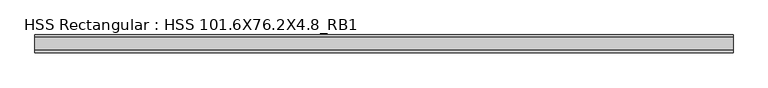
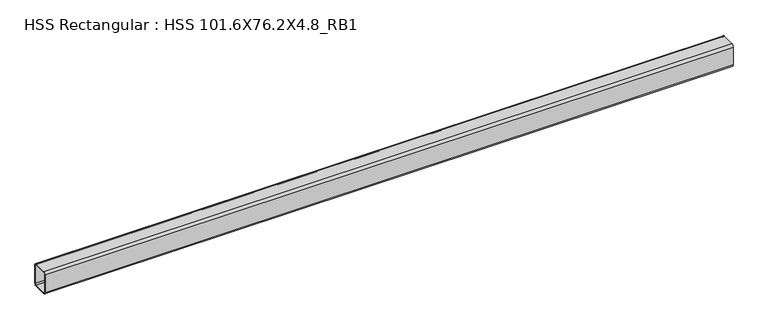
"""IFC4 building model written with IfcOpenShell, lengths in millimetres: beam geometry, HSS Rectangular : HSS 101.6X76.2X4.8_RB1."""

from ifc_helpers import new_model, si_unit, point, frame, frame_2d, origin, place, context, project, spatial, polyline, circle_curve, trimmed, segment, composite_curve, outline, extrude, source, transform, mapped, element, save


def hss_rectangular_hss_101_6x76_2x4_8_rb1_0456b7c3(model_context):
    return source(origin(), model_context, "Body", "SweptSolid", [
        extrude(outline(composite_curve([segment(trimmed(circle_curve(frame_2d((-28.575, 41.275)), 9.525), [point((-38.1, 41.275))], [point((-28.575, 50.8))], False, "CARTESIAN"), True, "CONTINUOUS"), segment(polyline([(-28.575, 50.8), (28.575, 50.8)]), True, "CONTINUOUS"), segment(trimmed(circle_curve(frame_2d((28.575, 41.275)), 9.525), [point((28.575, 50.8))], [point((38.1, 41.275))], False, "CARTESIAN"), True, "CONTINUOUS"), segment(polyline([(38.1, 41.275), (38.1, -41.275)]), True, "CONTINUOUS"), segment(trimmed(circle_curve(frame_2d((28.575, -41.275)), 9.525), [point((38.1, -41.275))], [point((28.575, -50.8))], False, "CARTESIAN"), True, "CONTINUOUS"), segment(polyline([(28.575, -50.8), (-28.575, -50.8)]), True, "CONTINUOUS"), segment(trimmed(circle_curve(frame_2d((-28.575, -41.275)), 9.525), [point((-28.575, -50.8))], [point((-38.1, -41.275))], False, "CARTESIAN"), True, "CONTINUOUS"), segment(polyline([(-38.1, -41.275), (-38.1, 41.275)]), True, "CONTINUOUS")], self_intersect=False), holes=[composite_curve([segment(polyline([(28.575, 46.0375), (-28.575, 46.0375)]), True, "CONTINUOUS"), segment(trimmed(circle_curve(frame_2d((-28.575, 41.275)), 4.7625), [point((-28.575, 46.0375))], [point((-33.3375, 41.275))], True, "CARTESIAN"), True, "CONTINUOUS"), segment(polyline([(-33.3375, 41.275), (-33.3375, -41.275)]), True, "CONTINUOUS"), segment(trimmed(circle_curve(frame_2d((-28.575, -41.275)), 4.7625), [point((-33.3375, -41.275))], [point((-28.575, -46.0375))], True, "CARTESIAN"), True, "CONTINUOUS"), segment(polyline([(-28.575, -46.0375), (28.575, -46.0375)]), True, "CONTINUOUS"), segment(trimmed(circle_curve(frame_2d((28.575, -41.275)), 4.7625), [point((28.575, -46.0375))], [point((33.3375, -41.275))], True, "CARTESIAN"), True, "CONTINUOUS"), segment(polyline([(33.3375, -41.275), (33.3375, 41.275)]), True, "CONTINUOUS"), segment(trimmed(circle_curve(frame_2d((28.575, 41.275)), 4.7625), [point((33.3375, 41.275))], [point((28.575, 46.0375))], True, "CARTESIAN"), True, "CONTINUOUS")], self_intersect=False)]), frame((-1527.8674477, 0.0, 0.0), z_axis=(1.0, 0.0, 0.0), x_axis=(0.0, 1.0, 0.0)), (0.0, 0.0, 1.0), 2998.5848947),
    ])


if __name__ == "__main__":
    model = new_model("IFC4")
    model_context = context("Model", 3, world=origin())
    ifc_project = project(units=[si_unit("LENGTHUNIT", "METRE", prefix="MILLI")], contexts=[model_context])
    site = spatial("IfcSite", under=ifc_project)
    building = spatial("IfcBuilding", under=site)
    placement = place(None, origin())
    hss_rectangular_hss_101_6x76_2x4_8_rb1_shape = hss_rectangular_hss_101_6x76_2x4_8_rb1_0456b7c3(model_context)
    element("IfcBeam", 1, ObjectType="HSS Rectangular : HSS 101.6X76.2X4.8_RB1", at=placement, inside=building, context=model_context, shape_type="MappedRepresentation", body=[
        mapped(hss_rectangular_hss_101_6x76_2x4_8_rb1_shape, transform((0.0, 0.0, 0.0), x_axis=(1.0, 0.0, 0.0), y_axis=(0.0, 1.0, 0.0), z_axis=(0.0, 0.0, 1.0))),
    ])
    save(model, "model.ifc")

# Revit data of these elements
# Type "HSS Rectangular : HSS 101.6X76.2X4.8_RB1"
#   Section Name Key = "HSS 4X3X3/16"
#   Assembly Code = "B10"
#   Width = 7.62 cm
#   Wall Nominal Thickness = 0.4763 cm
#   Wall Design Thickness = 0.442 cm
#   Torsional Moment of Inertia = 260.561 cm⁴
#   Torsional Modulus = 61.2876 cm³
#   Section Area = 14.4516 cm²
#   Plastic Modulus weak axis = 40.3122 cm³
#   Plastic Modulus strong axis = 49.1612 cm³
#   Perimeter = 0.881482 m²/m
#   Outer Fillet = 0.9525 cm
#   Nominal Weight = 12.1285 kgf/m
#   Moment of Inertia weak axis = 131.529 cm⁴
#   Moment of Inertia strong axis = 205.202 cm⁴
#   Inner Fillet = 0.4763 cm
#   Height = 10.16 cm
#   Elastic Modulus weak axis = 34.4128 cm³
#   Elastic Modulus strong axis = 40.476 cm³
#   Centroid Vertical = 5.08 cm
#   Centroid Horizontal = 3.81 cm
#   Length [instance default] = 1524 mm
#   Structural Material [instance default] = Steel ASTM A500, Grade B, Rectangular and Square
#   Principal Axes Angle = 0
# Element 1 (IfcBeam, "HSS Rectangular : HSS 101.6X76.2X4.8_RB1")
#   Structural Material = Steel ASTM A992
#   Materials on its faces: "Steel ASTM A992"
# Materials
#   "Steel ASTM A500, Grade B, Rectangular and Square": class "Metal", colour RGB 199 199 199, transparency 0, Description = "Carbon steel", Cost = 0
#   "Steel ASTM A992": class "Metal", colour RGB 199 199 199, transparency 0, Description = "Structural steel 50ksi", Cost = 0
